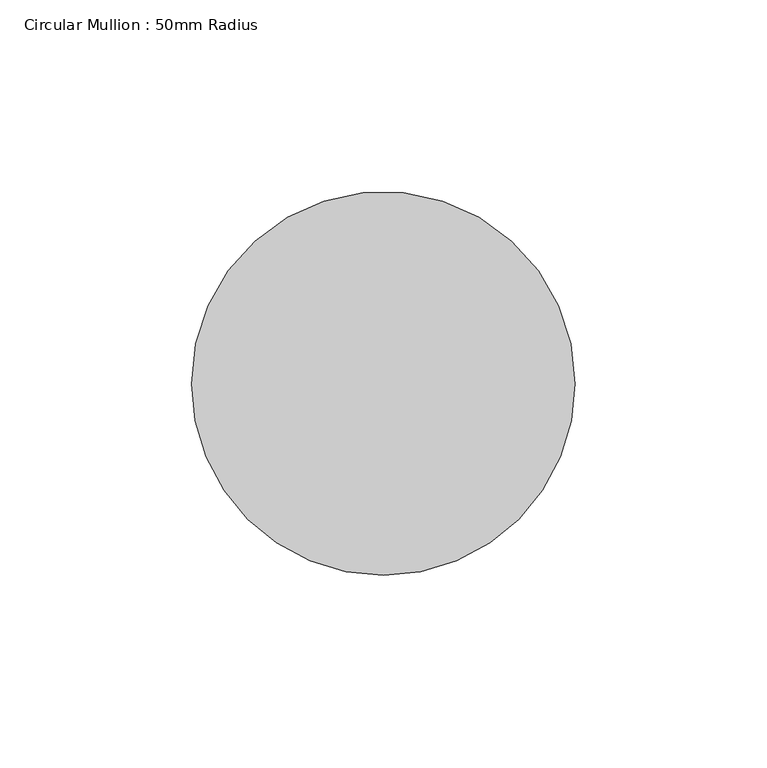
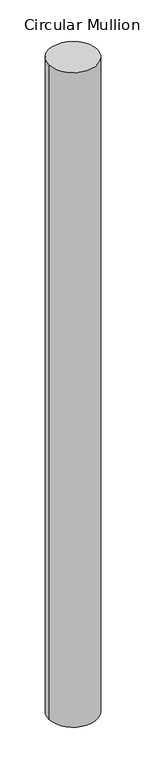
"""IFC4 building model written with IfcOpenShell, lengths in millimetres: member geometry, Circular Mullion : 50mm Radius."""

from ifc_helpers import new_model, si_unit, frame, origin, place, context, project, spatial, ellipse_curve, source, transform, mapped, element, save
from ifc_brep_helpers import plane_surface, cylinder_surface, advanced_brep


def circular_mullion_50mm_radius_9e4aa7c8(model_context):
    return source(origin(), model_context, "Body", "AdvancedBrep", [
        advanced_brep(
        [(-100.0, 0.0, 0.6757529), (0.0, 0.0, 0.0), (0.0, 0.0, -1431.5210404), (-100.0, 0.0, -1432.1547935)],
        [
            (0, 1, ellipse_curve(frame((-50.0, 0.0, 0.3378765), z_axis=(-0.0067566044461100675, -0.015101283103847446, -0.9998631404072142), x_axis=(-0.4083488092282802, -0.9126760375658072, 0.016543894796058417)), 50.0068439, 50.0)),
            (1, 2),
            (2, 3, ellipse_curve(frame((-50.0, 0.0, -1431.837917), z_axis=(-0.00633676809437141, -0.014162931946031212, 0.9998796211188676), x_axis=(0.408355540028511, 0.9126910811752428, 0.015515903814786142)), 50.0060197, 50.0)),
            (3, 0),
            (1, 0, ellipse_curve(frame((-50.0, 0.0, 0.3378765), z_axis=(-0.0067566044461100675, -0.015101283103847446, -0.9998631404072142), x_axis=(-0.4083488092282802, -0.9126760375658072, 0.016543894796058417)), 50.0068439, 50.0)),
            (3, 2, ellipse_curve(frame((-50.0, 0.0, -1431.837917), z_axis=(-0.00633676809437141, -0.014162931946031212, 0.9998796211188676), x_axis=(0.408355540028511, 0.9126910811752428, 0.015515903814786142)), 50.0060197, 50.0)),
        ],
        [
            cylinder_surface(frame((-50.0, 0.0, 0.0), z_axis=(0.0, 0.0, 1.0), x_axis=(1.0, 0.0, 0.0)), 50.0),
            plane_surface(frame((-278.2217336, 124.4817536, 0.0), z_axis=(0.006756604446110066, 0.015101283103847443, 0.999863140407214), x_axis=(0.4083488092282754, 0.912676037565809, -0.016543894796079386))),
            plane_surface(frame((-278.2217336, 124.4817536, -1431.5210404), z_axis=(0.00633676809437141, 0.014162931946031212, -0.9998796211188676), x_axis=(0.40835554002851093, 0.9126910811752427, 0.015515903814788068))),
        ],
        [
            (0, [[1, 2, 3, 4]]),
            (0, [[5, -4, 6, -2]]),
            (1, [[-1, -5]]),
            (2, [[-6, -3]]),
        ],
    ),
    ])


if __name__ == "__main__":
    model = new_model("IFC4")
    model_context = context("Model", 3, world=origin())
    ifc_project = project(units=[si_unit("LENGTHUNIT", "METRE", prefix="MILLI")], contexts=[model_context])
    site = spatial("IfcSite", under=ifc_project)
    building = spatial("IfcBuilding", under=site)
    placement = place(None, origin())
    circular_mullion_50mm_radius_shape = circular_mullion_50mm_radius_9e4aa7c8(model_context)
    element("IfcMember", 1, ObjectType="Circular Mullion : 50mm Radius", at=placement, inside=building, context=model_context, shape_type="MappedRepresentation", body=[
        mapped(circular_mullion_50mm_radius_shape, transform((0.0, 0.0, 0.0), x_axis=(1.0, 0.0, 0.0), y_axis=(0.0, 1.0, 0.0), z_axis=(0.0, 0.0, 1.0))),
    ])
    save(model, "model.ifc")

# Revit data of these elements
# Type "Circular Mullion : 50mm Radius"
#   built-in parameter 1007350 = 0.164042 (stored number, unit not read)
# Element 1 (IfcMember, "Circular Mullion : 50mm Radius")
#   Materials on its faces: "Aluminium"
# Materials
#   "Aluminium": class "Metal", colour RGB 247 247 247, transparency 0, Description = "Aluminium 6061", Cost = 0
